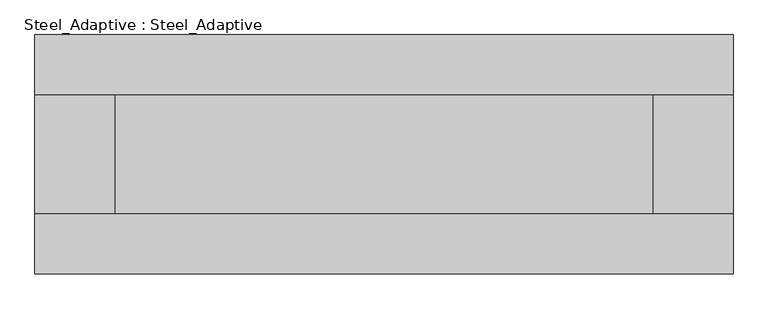
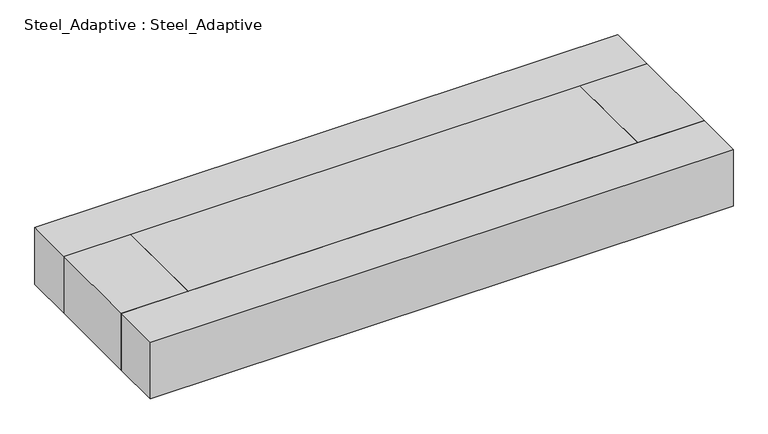
"""IFC4 building model written with IfcOpenShell, lengths in millimetres: proxy geometry, Steel_Adaptive : Steel_Adaptive."""

from ifc_helpers import new_model, si_unit, frame, origin, place, context, project, spatial, polyline, outline, extrude, source, transform, mapped, element, save


def steel_adaptive_steel_adaptive_804e0509(model_context):
    return source(origin(), model_context, "Body", "SweptSolid", [
        extrude(outline(polyline([(8750.0, 1500.0), (-8750.0, 1500.0), (-8750.0, 3000.0), (8750.0, 3000.0), (8750.0, 1500.0)])), frame((0.0, 0.0, 106900.0), z_axis=(0.0, 0.0, 1.0), x_axis=(1.0, 0.0, 0.0)), (0.0, 0.0, 1.0), 1800.0),
        extrude(outline(polyline([(-8750.0, -1500.0), (8750.0, -1500.0), (8750.0, -3000.0), (-8750.0, -3000.0), (-8750.0, -1500.0)])), frame((0.0, 0.0, 106900.0), z_axis=(0.0, 0.0, 1.0), x_axis=(1.0, 0.0, 0.0)), (0.0, 0.0, 1.0), 1800.0),
        extrude(outline(polyline([(6750.0, -1500.0), (6750.0, 1500.0), (8750.0, 1500.0), (8750.0, -1500.0), (6750.0, -1500.0)])), frame((0.0, 0.0, 106900.0), z_axis=(0.0, 0.0, 1.0), x_axis=(1.0, 0.0, 0.0)), (0.0, 0.0, 1.0), 1800.0),
        extrude(outline(polyline([(-6750.0, 1500.0), (-6750.0, -1500.0), (-8750.0, -1500.0), (-8750.0, 1500.0), (-6750.0, 1500.0)])), frame((0.0, 0.0, 106900.0), z_axis=(0.0, 0.0, 1.0), x_axis=(1.0, 0.0, 0.0)), (0.0, 0.0, 1.0), 1800.0),
        extrude(outline(polyline([(-6750.0, -1500.0), (-6750.0, 1500.0), (6750.0, 1500.0), (6750.0, -1500.0), (-6750.0, -1500.0)])), frame((0.0, 0.0, 106900.0), z_axis=(0.0, 0.0, 1.0), x_axis=(1.0, 0.0, 0.0)), (0.0, 0.0, 1.0), 1800.0),
    ])


if __name__ == "__main__":
    model = new_model("IFC4")
    model_context = context("Model", 3, world=origin())
    ifc_project = project(units=[si_unit("LENGTHUNIT", "METRE", prefix="MILLI")], contexts=[model_context])
    site = spatial("IfcSite", under=ifc_project)
    building = spatial("IfcBuilding", under=site)
    placement = place(None, origin())
    steel_adaptive_steel_adaptive_shape = steel_adaptive_steel_adaptive_804e0509(model_context)
    element("IfcBuildingElementProxy", 1, Name="Steel_Adaptive : Steel_Adaptive", ObjectType="Steel_Adaptive : Steel_Adaptive", at=placement, inside=building, context=model_context, shape_type="MappedRepresentation", body=[
        mapped(steel_adaptive_steel_adaptive_shape, transform((0.0, 0.0, 0.0), x_axis=(1.0, 0.0, 0.0), y_axis=(0.0, 1.0, 0.0), z_axis=(0.0, 0.0, 1.0))),
    ])
    save(model, "model.ifc")

# Revit data of these elements
# Type "Steel_Adaptive : Steel_Adaptive"
#   Width = 3000 mm
#   Top Width = 3000 mm
#   Length = 21000 mm
#   Height [instance default] = 80000 mm
#   Default Elevation = 0
# Element 1 (IfcBuildingElementProxy, "Steel_Adaptive : Steel_Adaptive")
#   Height = 106900 mm
